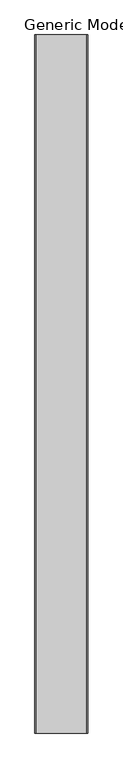
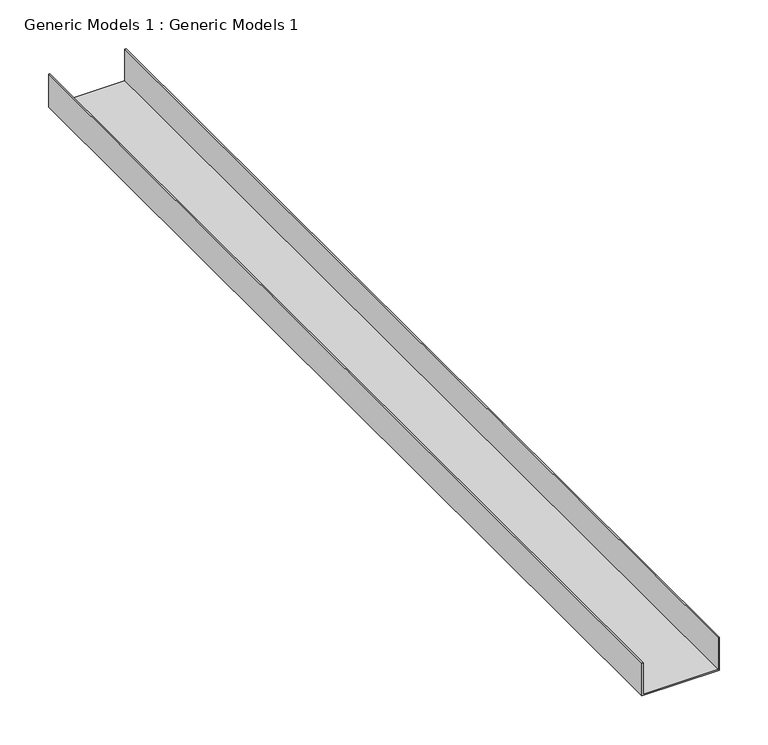
"""IFC4 building model written with IfcOpenShell, lengths in millimetres: proxy geometry, Generic Models 1 : Generic Models 1."""

from ifc_helpers import new_model, si_unit, frame, origin, place, context, project, spatial, polyline, outline, extrude, source, transform, mapped, element, save


def generic_models_1_generic_models_1_e7a28f78(model_context):
    return source(origin(), model_context, "Body", "SweptSolid", [
        extrude(outline(polyline([(0.0, 51003.2), (41.275, 51003.2), (41.275, 51001.6125), (1.5875, 51001.6125), (1.5875, 50912.7125), (41.275, 50912.7125), (41.275, 50911.125), (0.0, 50911.125), (0.0, 51003.2)])), frame((0.0, 0.0, 0.0), z_axis=(0.0, 1.0, 0.0), x_axis=(0.0, 0.0, 1.0)), (0.0, 0.0, 1.0), 1219.2),
    ])


if __name__ == "__main__":
    model = new_model("IFC4")
    model_context = context("Model", 3, world=origin())
    ifc_project = project(units=[si_unit("LENGTHUNIT", "METRE", prefix="MILLI")], contexts=[model_context])
    site = spatial("IfcSite", under=ifc_project)
    building = spatial("IfcBuilding", under=site)
    placement = place(None, origin())
    generic_models_1_generic_models_1_shape = generic_models_1_generic_models_1_e7a28f78(model_context)
    element("IfcBuildingElementProxy", 1, Name="Generic Models 1 : Generic Models 1", ObjectType="Generic Models 1 : Generic Models 1", at=placement, inside=building, context=model_context, shape_type="MappedRepresentation", body=[
        mapped(generic_models_1_generic_models_1_shape, transform((0.0, 0.0, 0.0), x_axis=(1.0, 0.0, 0.0), y_axis=(0.0, 1.0, 0.0), z_axis=(0.0, 0.0, 1.0))),
    ])
    save(model, "model.ifc")

# Revit data of these elements
# Element 1 (IfcBuildingElementProxy, "Generic Models 1 : Generic Models 1")
#   Materials on its faces: "METAL RUNNER ANCHORED TO STRUCTURE"
# Materials
#   "METAL RUNNER ANCHORED TO STRUCTURE": class "Unassigned", colour RGB 210 209 208, transparency 0, Keynote = "M05121300.02", Cost = 0
